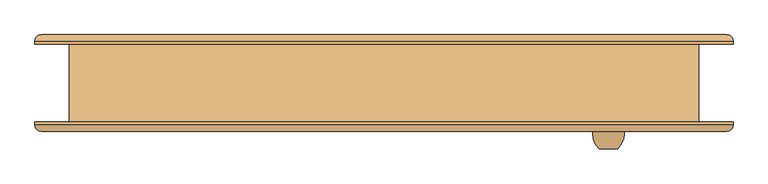
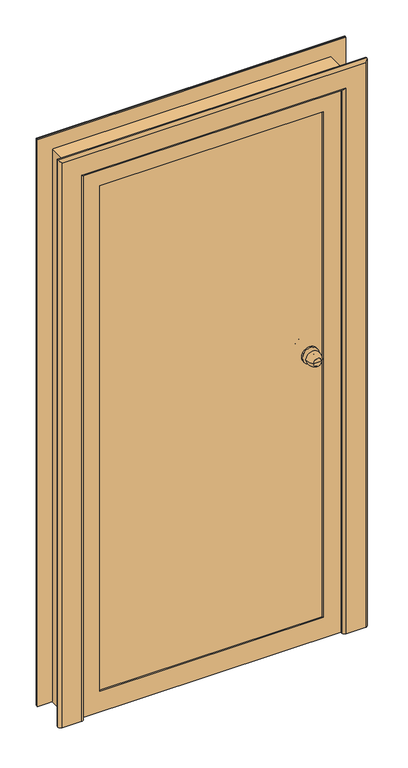
"""IFC4 building model written with IfcOpenShell, lengths in millimetres: door geometry, Наружная дверь 1-Навесная - Один проем наружу с порогом - 31173-2003 : ДСН КЛН  М1 УЗ 2100-1010 ГОСТ 31173-2003."""

from ifc_helpers import new_model, si_unit, point, frame, origin, place, context, project, spatial, polyline, circle_curve, ellipse_curve, trimmed, outline, extrude, faceted_brep, source, transform, mapped, element, save
from ifc_brep_helpers import plane_surface, cylinder_surface, revolved_surface, advanced_brep


def door_3e236f90(model_context):
    return source(origin(), model_context, "Body", "SolidModel", [
        advanced_brep(
        [(345.0, -105.5, 1100.0), (360.0, -105.5, 1100.0), (375.0, -105.5, 1100.0), (385.0, -75.5, 1100.0), (335.0, -75.5, 1100.0), (378.0, -75.5, 1100.0), (342.0, -75.5, 1100.0), (370.0, -67.5, 1100.0), (350.0, -67.5, 1100.0), (370.0, -61.5, 1100.0), (350.0, -61.5, 1100.0), (390.0, -61.5, 1100.0), (330.0, -61.5, 1100.0), (390.0, -55.5, 1100.0), (330.0, -55.5, 1100.0)],
        [
            (0, 1),
            (1, 2),
            (2, 0, circle_curve(frame((360.0, -105.5, 1100.0), z_axis=(0.0, -1.0, 0.0), x_axis=(1.0, 0.0, 0.0)), 15.0)),
            (0, 2, circle_curve(frame((360.0, -105.5, 1100.0), z_axis=(0.0, -1.0, 0.0), x_axis=(1.0, 0.0, 0.0)), 15.0)),
            (2, 3, circle_curve(frame((350.3773735, -80.6257912, 1100.0), z_axis=(0.0, 0.0, 1.0), x_axis=(-1.0, 0.0, 0.0)), 35.0)),
            (3, 4, circle_curve(frame((360.0, -75.5, 1100.0), z_axis=(0.0, -1.0, 0.0), x_axis=(1.0, 0.0, 0.0)), 25.0)),
            (4, 0, circle_curve(frame((369.6226265, -80.6257912, 1100.0), z_axis=(0.0, 0.0, 1.0), x_axis=(1.0, 0.0, 0.0)), 35.0)),
            (4, 3, circle_curve(frame((360.0, -75.5, 1100.0), z_axis=(0.0, -1.0, 0.0), x_axis=(1.0, 0.0, 0.0)), 25.0)),
            (3, 5),
            (5, 6, circle_curve(frame((360.0, -75.5, 1100.0), z_axis=(0.0, -1.0, 0.0), x_axis=(1.0, 0.0, 0.0)), 18.0)),
            (6, 4),
            (6, 5, circle_curve(frame((360.0, -75.5, 1100.0), z_axis=(0.0, -1.0, 0.0), x_axis=(1.0, 0.0, 0.0)), 18.0)),
            (5, 7, circle_curve(frame((378.0, -67.5, 1100.0), z_axis=(0.0, 0.0, -1.0), x_axis=(-1.0, 0.0, 0.0)), 8.0)),
            (7, 8, circle_curve(frame((360.0, -67.5, 1100.0), z_axis=(0.0, -1.0, 0.0), x_axis=(1.0, 0.0, 0.0)), 10.0)),
            (8, 6, circle_curve(frame((342.0, -67.5, 1100.0), z_axis=(0.0, 0.0, -1.0), x_axis=(1.0, 0.0, 0.0)), 8.0)),
            (8, 7, circle_curve(frame((360.0, -67.5, 1100.0), z_axis=(0.0, -1.0, 0.0), x_axis=(1.0, 0.0, 0.0)), 10.0)),
            (7, 9),
            (9, 10, circle_curve(frame((360.0, -61.5, 1100.0), z_axis=(0.0, -1.0, 0.0), x_axis=(1.0, 0.0, 0.0)), 10.0)),
            (10, 8),
            (10, 9, circle_curve(frame((360.0, -61.5, 1100.0), z_axis=(0.0, -1.0, 0.0), x_axis=(1.0, 0.0, 0.0)), 10.0)),
            (11, 12, circle_curve(frame((360.0, -61.5, 1100.0), z_axis=(0.0, -1.0, 0.0), x_axis=(-1.0, 0.0, 0.0)), 30.0)),
            (12, 11, circle_curve(frame((360.0, -61.5, 1100.0), z_axis=(0.0, -1.0, 0.0), x_axis=(-1.0, 0.0, 0.0)), 30.0)),
            (13, 14, circle_curve(frame((360.0, -55.5, 1100.0), z_axis=(0.0, 1.0, 0.0), x_axis=(-1.0, 0.0, 0.0)), 30.0)),
            (14, 13, circle_curve(frame((360.0, -55.5, 1100.0), z_axis=(0.0, 1.0, 0.0), x_axis=(-1.0, 0.0, 0.0)), 30.0)),
            (12, 14),
            (13, 11),
        ],
        [
            plane_surface(frame((360.0, -105.5, 1100.0), z_axis=(0.0, -1.0, 0.0), x_axis=(1.0, 0.0, 0.0))),
            revolved_surface(trimmed(ellipse_curve(frame((350.3773735, -80.6257912, 1100.0), z_axis=(0.0, 0.0, 1.0), x_axis=(-1.0, 0.0, 0.0)), 35.0, 35.0), [point((375.0, -105.5, 1100.0))], [point((385.0, -75.5, 1100.0))], True, "CARTESIAN"), (360.0, -135.5, 1100.0), (0.0, 1.0, 0.0)),
            plane_surface(frame((360.0, -75.5, 1100.0), z_axis=(0.0, 1.0, 0.0), x_axis=(1.0, 0.0, 0.0))),
            revolved_surface(trimmed(ellipse_curve(frame((378.0, -67.5, 1100.0), z_axis=(0.0, 0.0, -1.0), x_axis=(-1.0, 0.0, 0.0)), 8.0, 8.0), [point((378.0, -75.5, 1100.0))], [point((370.0, -67.5, 1100.0))], True, "CARTESIAN"), (360.0, -135.5, 1100.0), (0.0, 1.0, 0.0)),
            cylinder_surface(frame((360.0, -135.5, 1100.0), z_axis=(0.0, 1.0, 0.0), x_axis=(1.0, 0.0, 0.0)), 10.0),
            plane_surface(frame((330.0, -61.5, 1100.0), z_axis=(0.0, -1.0, 0.0), x_axis=(0.0, 0.0, 1.0))),
            plane_surface(frame((330.0, -55.5, 1100.0), z_axis=(0.0, 1.0, 0.0), x_axis=(0.0, 0.0, -1.0))),
            cylinder_surface(frame((360.0, -55.5, 1100.0), z_axis=(0.0, -1.0, 0.0), x_axis=(-1.0, 0.0, 0.0)), 30.0),
        ],
        [
            (0, [[1, 2, 3]]),
            (0, [[-1, 4, -2]]),
            (1, [[5, 6, 7, -3]]),
            (1, [[-7, 8, -5, -4]]),
            (2, [[9, 10, 11, -6]]),
            (2, [[-11, 12, -9, -8]]),
            (3, [[13, 14, 15, -10]]),
            (3, [[-15, 16, -13, -12]]),
            (4, [[17, 18, 19, -14]]),
            (4, [[-19, 20, -17, -16]]),
            (5, [[21, 22], [-20, -18]]),
            (6, [[23, 24]]),
            (7, [[25, -23, 26, -22]]),
            (7, [[-26, -24, -25, -21]]),
        ],
    ),
        advanced_brep(
        [(375.0, 64.5, 1100.0), (360.0, 64.5, 1100.0), (345.0, 64.5, 1100.0), (335.0, 34.5, 1100.0), (385.0, 34.5, 1100.0), (342.0, 34.5, 1100.0), (378.0, 34.5, 1100.0), (350.0, 26.5, 1100.0), (370.0, 26.5, 1100.0), (350.0, 20.5, 1100.0), (370.0, 20.5, 1100.0), (330.0, 20.5, 1100.0), (390.0, 20.5, 1100.0), (330.0, 14.5, 1100.0), (390.0, 14.5, 1100.0)],
        [
            (0, 1),
            (1, 2),
            (2, 0, circle_curve(frame((360.0, 64.5, 1100.0), z_axis=(0.0, 1.0, 0.0), x_axis=(-1.0, 0.0, 0.0)), 15.0)),
            (0, 2, circle_curve(frame((360.0, 64.5, 1100.0), z_axis=(0.0, 1.0, 0.0), x_axis=(-1.0, 0.0, 0.0)), 15.0)),
            (2, 3, circle_curve(frame((369.6226265, 39.6257912, 1100.0), z_axis=(0.0, 0.0, 1.0), x_axis=(1.0, 0.0, 0.0)), 35.0)),
            (3, 4, circle_curve(frame((360.0, 34.5, 1100.0), z_axis=(0.0, 1.0, 0.0), x_axis=(-1.0, 0.0, 0.0)), 25.0)),
            (4, 0, circle_curve(frame((350.3773735, 39.6257912, 1100.0), z_axis=(0.0, 0.0, 1.0), x_axis=(-1.0, 0.0, 0.0)), 35.0)),
            (4, 3, circle_curve(frame((360.0, 34.5, 1100.0), z_axis=(0.0, 1.0, 0.0), x_axis=(-1.0, 0.0, 0.0)), 25.0)),
            (3, 5),
            (5, 6, circle_curve(frame((360.0, 34.5, 1100.0), z_axis=(0.0, 1.0, 0.0), x_axis=(-1.0, 0.0, 0.0)), 18.0)),
            (6, 4),
            (6, 5, circle_curve(frame((360.0, 34.5, 1100.0), z_axis=(0.0, 1.0, 0.0), x_axis=(-1.0, 0.0, 0.0)), 18.0)),
            (5, 7, circle_curve(frame((342.0, 26.5, 1100.0), z_axis=(0.0, 0.0, -1.0), x_axis=(1.0, 0.0, 0.0)), 8.0)),
            (7, 8, circle_curve(frame((360.0, 26.5, 1100.0), z_axis=(0.0, 1.0, 0.0), x_axis=(-1.0, 0.0, 0.0)), 10.0)),
            (8, 6, circle_curve(frame((378.0, 26.5, 1100.0), z_axis=(0.0, 0.0, -1.0), x_axis=(-1.0, 0.0, 0.0)), 8.0)),
            (8, 7, circle_curve(frame((360.0, 26.5, 1100.0), z_axis=(0.0, 1.0, 0.0), x_axis=(-1.0, 0.0, 0.0)), 10.0)),
            (7, 9),
            (9, 10, circle_curve(frame((360.0, 20.5, 1100.0), z_axis=(0.0, 1.0, 0.0), x_axis=(-1.0, 0.0, 0.0)), 10.0)),
            (10, 8),
            (10, 9, circle_curve(frame((360.0, 20.5, 1100.0), z_axis=(0.0, 1.0, 0.0), x_axis=(-1.0, 0.0, 0.0)), 10.0)),
            (11, 12, circle_curve(frame((360.0, 20.5, 1100.0), z_axis=(0.0, 1.0, 0.0), x_axis=(1.0, 0.0, 0.0)), 30.0)),
            (12, 11, circle_curve(frame((360.0, 20.5, 1100.0), z_axis=(0.0, 1.0, 0.0), x_axis=(1.0, 0.0, 0.0)), 30.0)),
            (13, 14, circle_curve(frame((360.0, 14.5, 1100.0), z_axis=(0.0, -1.0, 0.0), x_axis=(1.0, 0.0, 0.0)), 30.0)),
            (14, 13, circle_curve(frame((360.0, 14.5, 1100.0), z_axis=(0.0, -1.0, 0.0), x_axis=(1.0, 0.0, 0.0)), 30.0)),
            (12, 14),
            (13, 11),
        ],
        [
            plane_surface(frame((360.0, 64.5, 1100.0), z_axis=(0.0, 1.0, 0.0), x_axis=(-1.0, 0.0, 0.0))),
            revolved_surface(trimmed(ellipse_curve(frame((369.6226265, 39.6257912, 1100.0), z_axis=(0.0, 0.0, 1.0), x_axis=(1.0, 0.0, 0.0)), 35.0, 35.0), [point((345.0, 64.5, 1100.0))], [point((335.0, 34.5, 1100.0))], True, "CARTESIAN"), (360.0, 94.5, 1100.0), (0.0, -1.0, 0.0)),
            plane_surface(frame((360.0, 34.5, 1100.0), z_axis=(0.0, -1.0, 0.0), x_axis=(-1.0, 0.0, 0.0))),
            revolved_surface(trimmed(ellipse_curve(frame((342.0, 26.5, 1100.0), z_axis=(0.0, 0.0, -1.0), x_axis=(1.0, 0.0, 0.0)), 8.0, 8.0), [point((342.0, 34.5, 1100.0))], [point((350.0, 26.5, 1100.0))], True, "CARTESIAN"), (360.0, 94.5, 1100.0), (0.0, -1.0, 0.0)),
            cylinder_surface(frame((360.0, 94.5, 1100.0), z_axis=(0.0, -1.0, 0.0), x_axis=(-1.0, 0.0, 0.0)), 10.0),
            plane_surface(frame((390.0, 20.5, 1100.0), z_axis=(0.0, 1.0, 0.0), x_axis=(0.0, 0.0, 1.0))),
            plane_surface(frame((390.0, 14.5, 1100.0), z_axis=(0.0, -1.0, 0.0), x_axis=(0.0, 0.0, -1.0))),
            cylinder_surface(frame((360.0, 14.5, 1100.0), z_axis=(0.0, 1.0, 0.0), x_axis=(1.0, 0.0, 0.0)), 30.0),
        ],
        [
            (0, [[1, 2, 3]]),
            (0, [[-1, 4, -2]]),
            (1, [[5, 6, 7, -3]]),
            (1, [[-7, 8, -5, -4]]),
            (2, [[9, 10, 11, -6]]),
            (2, [[-11, 12, -9, -8]]),
            (3, [[13, 14, 15, -10]]),
            (3, [[-15, 16, -13, -12]]),
            (4, [[17, 18, 19, -14]]),
            (4, [[-19, 20, -17, -16]]),
            (5, [[21, 22], [-20, -18]]),
            (6, [[23, 24]]),
            (7, [[25, -23, 26, -22]]),
            (7, [[-26, -24, -25, -21]]),
        ],
    ),
        faceted_brep([(440.0, 14.5, 42.0), (440.0, 9.5, 42.0), (-440.0, 9.5, 42.0), (-440.0, 14.5, 42.0), (440.0, 14.5, 2055.0), (440.0, 9.5, 2055.0), (-440.0, 9.5, 2055.0), (420.0, 9.5, 2035.0), (420.0, 9.5, 62.0), (-420.0, 9.5, 62.0), (-420.0, 9.5, 2035.0), (-440.0, 14.5, 2055.0), (420.0, -55.5, 2035.0), (420.0, -55.5, 62.0), (-420.0, -55.5, 62.0), (-420.0, -55.5, 2035.0)], [[[0, 1, 2, 3]], [[4, 5, 1, 0]], [[5, 6, 2, 1], [7, 8, 9, 10]], [[2, 6, 11, 3]], [[11, 4, 0, 3]], [[7, 12, 13, 8]], [[9, 8, 13, 14]], [[15, 10, 9, 14]], [[12, 15, 14, 13]], [[4, 11, 6, 5]], [[7, 10, 15, 12]]]),
        extrude(outline(polyline([(0.0, 470.0), (0.0, 485.0), (2100.0, 485.0), (2100.0, -485.0), (0.0, -485.0), (0.0, -470.0), (2085.0, -470.0), (2085.0, 470.0), (0.0, 470.0)])), frame((0.0, 7.5, 0.0), z_axis=(0.0, 1.0, 0.0), x_axis=(0.0, 0.0, 1.0)), (0.0, 0.0, 1.0), 55.0),
        faceted_brep([(485.0, 7.5, 0.0), (485.0, -62.5, 0.0), (-485.0, -62.5, 0.0), (-485.0, 7.5, 0.0), (-485.0, -62.5, 2100.0), (-485.0, 7.5, 2100.0), (485.0, -62.5, 2100.0), (-405.0, -62.5, 2020.0), (405.0, -62.5, 2020.0), (405.0, -62.5, 80.0), (-405.0, -62.5, 80.0), (485.0, 7.5, 2100.0), (-425.0, 7.5, 60.0), (425.0, 7.5, 60.0), (425.0, 7.5, 2040.0), (-425.0, 7.5, 2040.0), (425.0, -57.5, 60.0), (-425.0, -57.5, 60.0), (-425.0, -57.5, 2040.0), (425.0, -57.5, 2040.0), (-405.0, -57.5, 80.0), (405.0, -57.5, 80.0), (405.0, -57.5, 2020.0), (-405.0, -57.5, 2020.0)], [[[0, 1, 2, 3]], [[3, 2, 4, 5]], [[2, 1, 6, 4], [7, 8, 9, 10]], [[5, 11, 0, 3], [12, 13, 14, 15]], [[16, 13, 12, 17]], [[17, 12, 15, 18]], [[18, 19, 16, 17], [20, 21, 22, 23]], [[9, 21, 20, 10]], [[10, 20, 23, 7]], [[11, 6, 1, 0]], [[19, 14, 13, 16]], [[8, 22, 21, 9]], [[5, 4, 6, 11]], [[18, 15, 14, 19]], [[7, 23, 22, 8]]]),
        advanced_brep(
        [(-560.0, -62.5, 0.0), (-470.0, -62.5, 0.0), (-470.0, -67.5, 0.0), (-480.0, -77.5, 0.0), (-550.0, -77.5, 0.0), (-560.0, -67.5, 0.0), (-560.0, -62.5, 2175.0), (560.0, -62.5, 2175.0), (560.0, -62.5, 0.0), (470.0, -62.5, 0.0), (470.0, -62.5, 2085.0), (-470.0, -62.5, 2085.0), (-470.0, -67.5, 2085.0), (-480.0, -77.5, 2095.0), (480.0, -77.5, 2095.0), (480.0, -77.5, 0.0), (550.0, -77.5, 0.0), (550.0, -77.5, 2165.0), (-550.0, -77.5, 2165.0), (-560.0, -67.5, 2175.0), (560.0, -67.5, 2175.0), (560.0, -67.5, 0.0), (470.0, -67.5, 0.0), (470.0, -67.5, 2085.0)],
        [
            (0, 1),
            (1, 2),
            (2, 3, circle_curve(frame((-480.0, -67.5, 0.0), z_axis=(0.0, 0.0, -1.0), x_axis=(-1.0, 0.0, 0.0)), 10.0)),
            (3, 4),
            (4, 5, circle_curve(frame((-550.0, -67.5, 0.0), z_axis=(0.0, 0.0, -1.0), x_axis=(-1.0, 0.0, 0.0)), 10.0)),
            (5, 0),
            (0, 6),
            (6, 7),
            (7, 8),
            (8, 9),
            (9, 10),
            (10, 11),
            (11, 1),
            (11, 12),
            (12, 2),
            (12, 13, ellipse_curve(frame((-480.0, -67.5, 2095.0), z_axis=(-0.7071067811865475, 0.0, -0.7071067811865475), x_axis=(0.7071067811865474, 0.0, -0.7071067811865476)), 14.1421356, 10.0)),
            (13, 3),
            (13, 14),
            (14, 15),
            (15, 16),
            (16, 17),
            (17, 18),
            (18, 4),
            (18, 19, ellipse_curve(frame((-550.0, -67.5, 2165.0), z_axis=(-0.7071067811865475, 0.0, -0.7071067811865475), x_axis=(0.7071067811865474, 0.0, -0.7071067811865476)), 14.1421356, 10.0)),
            (19, 5),
            (19, 6),
            (7, 20),
            (20, 21),
            (21, 8),
            (21, 16, circle_curve(frame((550.0, -67.5, 0.0), z_axis=(0.0, 0.0, -1.0), x_axis=(1.0, 0.0, 0.0)), 10.0)),
            (15, 22, circle_curve(frame((480.0, -67.5, 0.0), z_axis=(0.0, 0.0, -1.0), x_axis=(1.0, 0.0, 0.0)), 10.0)),
            (22, 9),
            (23, 10),
            (22, 23),
            (14, 23, ellipse_curve(frame((480.0, -67.5, 2095.0), z_axis=(0.7071067811865475, 0.0, -0.7071067811865475), x_axis=(0.7071067811865474, 0.0, 0.7071067811865476)), 14.1421356, 10.0)),
            (20, 17, ellipse_curve(frame((550.0, -67.5, 2165.0), z_axis=(0.7071067811865475, 0.0, -0.7071067811865475), x_axis=(0.7071067811865474, 0.0, 0.7071067811865476)), 14.1421356, 10.0)),
            (23, 12),
            (20, 19),
        ],
        [
            plane_surface(frame((-505.0, -62.5, 0.0), z_axis=(0.0, 0.0, -1.0), x_axis=(0.0, -1.0, 0.0))),
            plane_surface(frame((-560.0, -62.5, 0.0), z_axis=(0.0, 1.0, 0.0), x_axis=(0.0, 0.0, 1.0))),
            plane_surface(frame((-470.0, -62.5, 0.0), z_axis=(1.0, 0.0, 0.0), x_axis=(0.0, 0.0, 1.0))),
            cylinder_surface(frame((-480.0, -67.5, 0.0), z_axis=(0.0, 0.0, -1.0), x_axis=(-1.0, 0.0, 0.0)), 10.0),
            plane_surface(frame((-480.0, -77.5, 0.0), z_axis=(0.0, -1.0, 0.0), x_axis=(0.0, 0.0, 1.0))),
            cylinder_surface(frame((-550.0, -67.5, 0.0), z_axis=(0.0, 0.0, -1.0), x_axis=(-1.0, 0.0, 0.0)), 10.0),
            plane_surface(frame((-560.0, -67.5, 0.0), z_axis=(-1.0, 0.0, 0.0), x_axis=(0.0, 0.0, 1.0))),
            plane_surface(frame((560.0, -67.5, 2175.0), z_axis=(1.0, 0.0, 0.0), x_axis=(0.0, 0.0, -1.0))),
            plane_surface(frame((505.0, -62.5, 0.0), z_axis=(0.0, 0.0, -1.0), x_axis=(0.0, -1.0, 0.0))),
            plane_surface(frame((470.0, -62.5, 2085.0), z_axis=(-1.0, 0.0, 0.0), x_axis=(0.0, 0.0, -1.0))),
            cylinder_surface(frame((480.0, -67.5, 2120.0), z_axis=(0.0, 0.0, 1.0), x_axis=(1.0, 0.0, 0.0)), 10.0),
            cylinder_surface(frame((550.0, -67.5, 2120.0), z_axis=(0.0, 0.0, 1.0), x_axis=(1.0, 0.0, 0.0)), 10.0),
            plane_surface(frame((-470.0, -62.5, 2085.0), z_axis=(0.0, 0.0, -1.0), x_axis=(1.0, 0.0, 0.0))),
            cylinder_surface(frame((-505.0, -67.5, 2095.0), z_axis=(-1.0, 0.0, 0.0), x_axis=(0.0, 0.0, 1.0)), 10.0),
            cylinder_surface(frame((-505.0, -67.5, 2165.0), z_axis=(-1.0, 0.0, 0.0), x_axis=(0.0, 0.0, 1.0)), 10.0),
            plane_surface(frame((-560.0, -67.5, 2175.0), z_axis=(0.0, 0.0, 1.0), x_axis=(1.0, 0.0, 0.0))),
        ],
        [
            (0, [[1, 2, 3, 4, 5, 6]]),
            (1, [[-1, 7, 8, 9, 10, 11, 12, 13]]),
            (2, [[-2, -13, 14, 15]]),
            (3, [[-3, -15, 16, 17]]),
            (4, [[-4, -17, 18, 19, 20, 21, 22, 23]]),
            (5, [[-5, -23, 24, 25]]),
            (6, [[-6, -25, 26, -7]]),
            (7, [[27, 28, 29, -9]]),
            (8, [[-29, 30, -20, 31, 32, -10]]),
            (9, [[33, -11, -32, 34]]),
            (10, [[35, -34, -31, -19]]),
            (11, [[36, -21, -30, -28]]),
            (12, [[-14, -12, -33, 37]]),
            (13, [[-16, -37, -35, -18]]),
            (14, [[-24, -22, -36, 38]]),
            (15, [[-26, -38, -27, -8]]),
        ],
    ),
        advanced_brep(
        [(560.0, 62.5, 0.0), (470.0, 62.5, 0.0), (470.0, 67.5, 0.0), (480.0, 77.5, 0.0), (550.0, 77.5, 0.0), (560.0, 67.5, 0.0), (560.0, 62.5, 2175.0), (-560.0, 62.5, 2175.0), (-560.0, 62.5, 0.0), (-470.0, 62.5, 0.0), (-470.0, 62.5, 2085.0), (470.0, 62.5, 2085.0), (470.0, 67.5, 2085.0), (480.0, 77.5, 2095.0), (-480.0, 77.5, 2095.0), (-480.0, 77.5, 0.0), (-550.0, 77.5, 0.0), (-550.0, 77.5, 2165.0), (550.0, 77.5, 2165.0), (560.0, 67.5, 2175.0), (-560.0, 67.5, 2175.0), (-560.0, 67.5, 0.0), (-470.0, 67.5, 0.0), (-470.0, 67.5, 2085.0)],
        [
            (0, 1),
            (1, 2),
            (2, 3, circle_curve(frame((480.0, 67.5, 0.0), z_axis=(0.0, 0.0, -1.0), x_axis=(1.0, 0.0, 0.0)), 10.0)),
            (3, 4),
            (4, 5, circle_curve(frame((550.0, 67.5, 0.0), z_axis=(0.0, 0.0, -1.0), x_axis=(1.0, 0.0, 0.0)), 10.0)),
            (5, 0),
            (0, 6),
            (6, 7),
            (7, 8),
            (8, 9),
            (9, 10),
            (10, 11),
            (11, 1),
            (11, 12),
            (12, 2),
            (12, 13, ellipse_curve(frame((480.0, 67.5, 2095.0), z_axis=(0.7071067811865475, 0.0, -0.7071067811865475), x_axis=(-0.7071067811865474, 0.0, -0.7071067811865476)), 14.1421356, 10.0)),
            (13, 3),
            (13, 14),
            (14, 15),
            (15, 16),
            (16, 17),
            (17, 18),
            (18, 4),
            (18, 19, ellipse_curve(frame((550.0, 67.5, 2165.0), z_axis=(0.7071067811865475, 0.0, -0.7071067811865475), x_axis=(-0.7071067811865474, 0.0, -0.7071067811865476)), 14.1421356, 10.0)),
            (19, 5),
            (19, 6),
            (7, 20),
            (20, 21),
            (21, 8),
            (21, 16, circle_curve(frame((-550.0, 67.5, 0.0), z_axis=(0.0, 0.0, -1.0), x_axis=(-1.0, 0.0, 0.0)), 10.0)),
            (15, 22, circle_curve(frame((-480.0, 67.5, 0.0), z_axis=(0.0, 0.0, -1.0), x_axis=(-1.0, 0.0, 0.0)), 10.0)),
            (22, 9),
            (23, 10),
            (22, 23),
            (14, 23, ellipse_curve(frame((-480.0, 67.5, 2095.0), z_axis=(-0.7071067811865475, 0.0, -0.7071067811865475), x_axis=(-0.7071067811865474, 0.0, 0.7071067811865476)), 14.1421356, 10.0)),
            (20, 17, ellipse_curve(frame((-550.0, 67.5, 2165.0), z_axis=(-0.7071067811865475, 0.0, -0.7071067811865475), x_axis=(-0.7071067811865474, 0.0, 0.7071067811865476)), 14.1421356, 10.0)),
            (23, 12),
            (20, 19),
        ],
        [
            plane_surface(frame((505.0, 62.5, 0.0), z_axis=(0.0, 0.0, -1.0), x_axis=(0.0, -1.0, 0.0))),
            plane_surface(frame((560.0, 62.5, 0.0), z_axis=(0.0, -1.0, 0.0), x_axis=(0.0, 0.0, 1.0))),
            plane_surface(frame((470.0, 62.5, 0.0), z_axis=(-1.0, 0.0, 0.0), x_axis=(0.0, 0.0, 1.0))),
            cylinder_surface(frame((480.0, 67.5, 0.0), z_axis=(0.0, 0.0, -1.0), x_axis=(1.0, 0.0, 0.0)), 10.0),
            plane_surface(frame((480.0, 77.5, 0.0), z_axis=(0.0, 1.0, 0.0), x_axis=(0.0, 0.0, 1.0))),
            cylinder_surface(frame((550.0, 67.5, 0.0), z_axis=(0.0, 0.0, -1.0), x_axis=(1.0, 0.0, 0.0)), 10.0),
            plane_surface(frame((560.0, 67.5, 0.0), z_axis=(1.0, 0.0, 0.0), x_axis=(0.0, 0.0, 1.0))),
            plane_surface(frame((-560.0, 67.5, 2175.0), z_axis=(-1.0, 0.0, 0.0), x_axis=(0.0, 0.0, -1.0))),
            plane_surface(frame((-505.0, 62.5, 0.0), z_axis=(0.0, 0.0, -1.0), x_axis=(0.0, -1.0, 0.0))),
            plane_surface(frame((-470.0, 62.5, 2085.0), z_axis=(1.0, 0.0, 0.0), x_axis=(0.0, 0.0, -1.0))),
            cylinder_surface(frame((-480.0, 67.5, 2120.0), z_axis=(0.0, 0.0, 1.0), x_axis=(-1.0, 0.0, 0.0)), 10.0),
            cylinder_surface(frame((-550.0, 67.5, 2120.0), z_axis=(0.0, 0.0, 1.0), x_axis=(-1.0, 0.0, 0.0)), 10.0),
            plane_surface(frame((470.0, 62.5, 2085.0), z_axis=(0.0, 0.0, -1.0), x_axis=(-1.0, 0.0, 0.0))),
            cylinder_surface(frame((505.0, 67.5, 2095.0), z_axis=(1.0, 0.0, 0.0), x_axis=(0.0, 0.0, 1.0)), 10.0),
            cylinder_surface(frame((505.0, 67.5, 2165.0), z_axis=(1.0, 0.0, 0.0), x_axis=(0.0, 0.0, 1.0)), 10.0),
            plane_surface(frame((560.0, 67.5, 2175.0), z_axis=(0.0, 0.0, 1.0), x_axis=(-1.0, 0.0, 0.0))),
        ],
        [
            (0, [[1, 2, 3, 4, 5, 6]]),
            (1, [[-1, 7, 8, 9, 10, 11, 12, 13]]),
            (2, [[-2, -13, 14, 15]]),
            (3, [[-3, -15, 16, 17]]),
            (4, [[-4, -17, 18, 19, 20, 21, 22, 23]]),
            (5, [[-5, -23, 24, 25]]),
            (6, [[-6, -25, 26, -7]]),
            (7, [[27, 28, 29, -9]]),
            (8, [[-29, 30, -20, 31, 32, -10]]),
            (9, [[33, -11, -32, 34]]),
            (10, [[35, -34, -31, -19]]),
            (11, [[36, -21, -30, -28]]),
            (12, [[-14, -12, -33, 37]]),
            (13, [[-16, -37, -35, -18]]),
            (14, [[-24, -22, -36, 38]]),
            (15, [[-26, -38, -27, -8]]),
        ],
    ),
        extrude(outline(polyline([(0.0, 485.0), (0.0, 505.0), (2120.0, 505.0), (2120.0, -505.0), (0.0, -505.0), (0.0, -485.0), (2100.0, -485.0), (2100.0, 485.0), (0.0, 485.0)])), frame((0.0, -62.5, 0.0), z_axis=(0.0, 1.0, 0.0), x_axis=(0.0, 0.0, 1.0)), (0.0, 0.0, 1.0), 125.0),
    ])


if __name__ == "__main__":
    model = new_model("IFC4")
    model_context = context("Model", 3, world=origin())
    ifc_project = project(units=[si_unit("LENGTHUNIT", "METRE", prefix="MILLI")], contexts=[model_context])
    site = spatial("IfcSite", under=ifc_project)
    building = spatial("IfcBuilding", under=site)
    placement = place(None, origin())
    door_shape = door_3e236f90(model_context)
    element("IfcDoor", 1, ObjectType="Наружная дверь 1-Навесная - Один проем наружу с порогом - 31173-2003 : ДСН КЛН  М1 УЗ 2100-1010 ГОСТ 31173-2003", at=placement, inside=building, context=model_context, shape_type="MappedRepresentation", body=[
        mapped(door_shape, transform((0.0, 0.0, 0.0), x_axis=(1.0, 0.0, 0.0), y_axis=(0.0, 1.0, 0.0), z_axis=(0.0, 0.0, 1.0))),
    ])
    save(model, "model.ifc")

# Revit data of these elements
# Type "Наружная дверь 1-Навесная - Один проем наружу с порогом - 31173-2003 : ДСН КЛН  М1 УЗ 2100-1010 ГОСТ 31173-2003"
#   Type Mark = "148"
#   Description = "ДСН КЛН  М1 УЗ 2100-900 ГОСТ 31173-2003"
#   Проекционное соединение по ширине = 90 mm
#   Rough Width = 1010 mm
#   Rough Height = 2120 mm
#   Угол проема [instance default] = 30°
#   Толщина_Тепл_Изоляции = 20 mm
#   Heat Transfer Coefficient (U) = 3.7021 W/(m²·K)
#   Height = 2100 mm
#   Width = 970 mm
#   Ширина каркаса = 60 mm
#   Толщина каркаса = 70 mm
#   Вставка двери [instance default] = 0 mm
#   Правая сторона = no
#   Левая сторона = yes
#   Function = 1
#   Обрезка = Сталь
#   Панель = Сталь
#   Тепловая изоляция = Тепловая изоляция
#   Кадр = Сталь
#   Дверная ручка = Металл
#   Visual Light Transmittance = 0
#   Solar Heat Gain Coefficient = 0
#   Construction Type Id = ""
#   Wall Closure = (empty or 0)
#   Analytic Construction = (empty or 0)
# Element 1 (IfcDoor, "Наружная дверь 1-Навесная - Один проем наружу с порогом - 31173-2003 : ДСН КЛН  М1 УЗ 2100-1010 ГОСТ 31173-2003")
#   Materials on its faces: "Сталь", "Металл", "Тепловая изоляция"
# Materials
#   "Сталь": class "Металл", colour RGB 247 247 247, transparency 0
#   "Тепловая изоляция": class "Пластмасса", colour RGB 185 154 119, transparency 0, Cost = 0
#   "Металл": class "Металл", colour RGB 249 249 249, transparency 0
